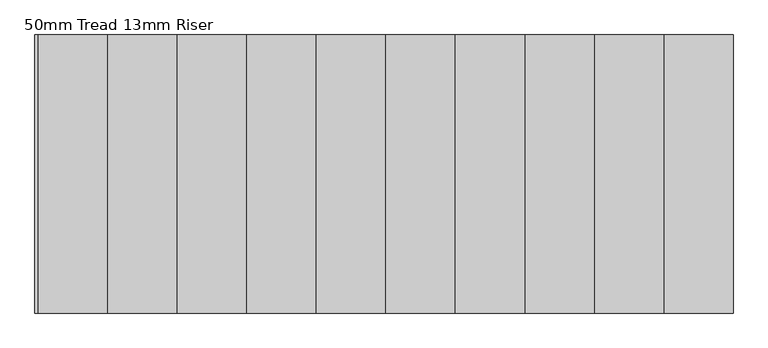
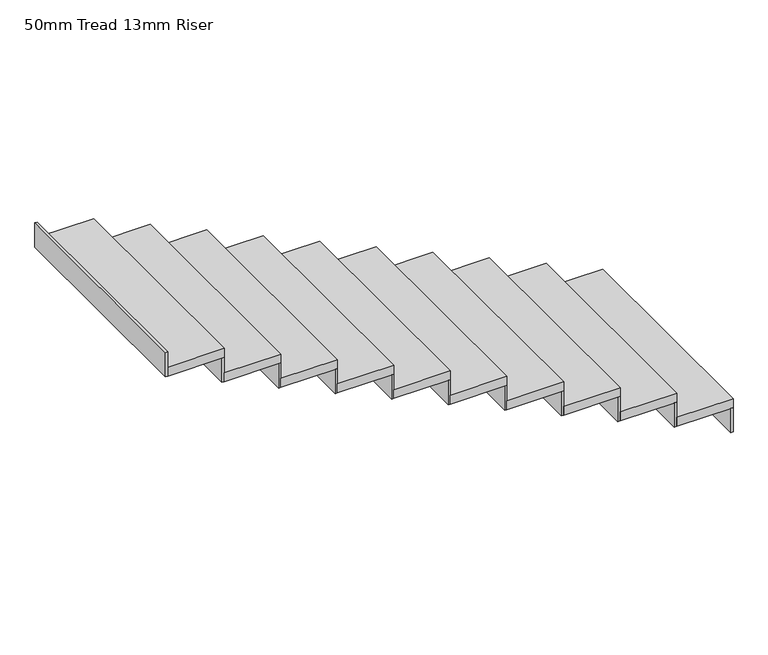
"""IFC4 building model written with IfcOpenShell, lengths in millimetres: stair flight geometry, 50mm Tread 13mm Riser."""

from ifc_helpers import new_model, si_unit, frame, origin, place, context, project, spatial, polyline, outline, extrude, source, transform, mapped, element, save


def stair_flight_50mm_tread_13mm_riser_e41575d0(model_context):
    return source(origin(), model_context, "Body", "SweptSolid", [
        extrude(outline(polyline([(20726.9907974, -2493.8863261), (20739.4907974, -2493.8863261), (20739.4907974, -3693.8863261), (20726.9907974, -3693.8863261), (20726.9907974, -2493.8863261)])), frame((0.0, 0.0, 1450.0), z_axis=(0.0, 0.0, 1.0), x_axis=(1.0, 0.0, 0.0)), (0.0, 0.0, 1.0), 136.3636364),
        extrude(outline(polyline([(20439.4907974, -3693.8863261), (20439.4907974, -2493.8863261), (20739.4907974, -2493.8863261), (20739.4907974, -3693.8863261), (20439.4907974, -3693.8863261)])), frame((0.0, 0.0, 1586.3636364), z_axis=(0.0, 0.0, 1.0), x_axis=(1.0, 0.0, 0.0)), (0.0, 0.0, 1.0), 50.0),
        extrude(outline(polyline([(20426.9907974, -2493.8863261), (20439.4907974, -2493.8863261), (20439.4907974, -3693.8863261), (20426.9907974, -3693.8863261), (20426.9907974, -2493.8863261)])), frame((0.0, 0.0, 1586.3636364), z_axis=(0.0, 0.0, 1.0), x_axis=(1.0, 0.0, 0.0)), (0.0, 0.0, 1.0), 136.3636364),
        extrude(outline(polyline([(20139.4907974, -3693.8863261), (20139.4907974, -2493.8863261), (20439.4907974, -2493.8863261), (20439.4907974, -3693.8863261), (20139.4907974, -3693.8863261)])), frame((0.0, 0.0, 1722.7272727), z_axis=(0.0, 0.0, 1.0), x_axis=(1.0, 0.0, 0.0)), (0.0, 0.0, 1.0), 50.0),
        extrude(outline(polyline([(20126.9907974, -2493.8863261), (20139.4907974, -2493.8863261), (20139.4907974, -3693.8863261), (20126.9907974, -3693.8863261), (20126.9907974, -2493.8863261)])), frame((0.0, 0.0, 1722.7272727), z_axis=(0.0, 0.0, 1.0), x_axis=(1.0, 0.0, 0.0)), (0.0, 0.0, 1.0), 136.3636364),
        extrude(outline(polyline([(19839.4907974, -3693.8863261), (19839.4907974, -2493.8863261), (20139.4907974, -2493.8863261), (20139.4907974, -3693.8863261), (19839.4907974, -3693.8863261)])), frame((0.0, 0.0, 1859.0909091), z_axis=(0.0, 0.0, 1.0), x_axis=(1.0, 0.0, 0.0)), (0.0, 0.0, 1.0), 50.0),
        extrude(outline(polyline([(19826.9907974, -2493.8863261), (19839.4907974, -2493.8863261), (19839.4907974, -3693.8863261), (19826.9907974, -3693.8863261), (19826.9907974, -2493.8863261)])), frame((0.0, 0.0, 1859.0909091), z_axis=(0.0, 0.0, 1.0), x_axis=(1.0, 0.0, 0.0)), (0.0, 0.0, 1.0), 136.3636364),
        extrude(outline(polyline([(19539.4907974, -3693.8863261), (19539.4907974, -2493.8863261), (19839.4907974, -2493.8863261), (19839.4907974, -3693.8863261), (19539.4907974, -3693.8863261)])), frame((0.0, 0.0, 1995.4545455), z_axis=(0.0, 0.0, 1.0), x_axis=(1.0, 0.0, 0.0)), (0.0, 0.0, 1.0), 50.0),
        extrude(outline(polyline([(19526.9907974, -2493.8863261), (19539.4907974, -2493.8863261), (19539.4907974, -3693.8863261), (19526.9907974, -3693.8863261), (19526.9907974, -2493.8863261)])), frame((0.0, 0.0, 1995.4545455), z_axis=(0.0, 0.0, 1.0), x_axis=(1.0, 0.0, 0.0)), (0.0, 0.0, 1.0), 136.3636364),
        extrude(outline(polyline([(19239.4907974, -3693.8863261), (19239.4907974, -2493.8863261), (19539.4907974, -2493.8863261), (19539.4907974, -3693.8863261), (19239.4907974, -3693.8863261)])), frame((0.0, 0.0, 2131.8181818), z_axis=(0.0, 0.0, 1.0), x_axis=(1.0, 0.0, 0.0)), (0.0, 0.0, 1.0), 50.0),
        extrude(outline(polyline([(19226.9907974, -2493.8863261), (19239.4907974, -2493.8863261), (19239.4907974, -3693.8863261), (19226.9907974, -3693.8863261), (19226.9907974, -2493.8863261)])), frame((0.0, 0.0, 2131.8181818), z_axis=(0.0, 0.0, 1.0), x_axis=(1.0, 0.0, 0.0)), (0.0, 0.0, 1.0), 136.3636364),
        extrude(outline(polyline([(18939.4907974, -3693.8863261), (18939.4907974, -2493.8863261), (19239.4907974, -2493.8863261), (19239.4907974, -3693.8863261), (18939.4907974, -3693.8863261)])), frame((0.0, 0.0, 2268.1818182), z_axis=(0.0, 0.0, 1.0), x_axis=(1.0, 0.0, 0.0)), (0.0, 0.0, 1.0), 50.0),
        extrude(outline(polyline([(18926.9907974, -2493.8863261), (18939.4907974, -2493.8863261), (18939.4907974, -3693.8863261), (18926.9907974, -3693.8863261), (18926.9907974, -2493.8863261)])), frame((0.0, 0.0, 2268.1818182), z_axis=(0.0, 0.0, 1.0), x_axis=(1.0, 0.0, 0.0)), (0.0, 0.0, 1.0), 136.3636364),
        extrude(outline(polyline([(18639.4907974, -3693.8863261), (18639.4907974, -2493.8863261), (18939.4907974, -2493.8863261), (18939.4907974, -3693.8863261), (18639.4907974, -3693.8863261)])), frame((0.0, 0.0, 2404.5454545), z_axis=(0.0, 0.0, 1.0), x_axis=(1.0, 0.0, 0.0)), (0.0, 0.0, 1.0), 50.0),
        extrude(outline(polyline([(18626.9907974, -2493.8863261), (18639.4907974, -2493.8863261), (18639.4907974, -3693.8863261), (18626.9907974, -3693.8863261), (18626.9907974, -2493.8863261)])), frame((0.0, 0.0, 2404.5454545), z_axis=(0.0, 0.0, 1.0), x_axis=(1.0, 0.0, 0.0)), (0.0, 0.0, 1.0), 136.3636364),
        extrude(outline(polyline([(18339.4907974, -3693.8863261), (18339.4907974, -2493.8863261), (18639.4907974, -2493.8863261), (18639.4907974, -3693.8863261), (18339.4907974, -3693.8863261)])), frame((0.0, 0.0, 2540.9090909), z_axis=(0.0, 0.0, 1.0), x_axis=(1.0, 0.0, 0.0)), (0.0, 0.0, 1.0), 50.0),
        extrude(outline(polyline([(18326.9907974, -2493.8863261), (18339.4907974, -2493.8863261), (18339.4907974, -3693.8863261), (18326.9907974, -3693.8863261), (18326.9907974, -2493.8863261)])), frame((0.0, 0.0, 2540.9090909), z_axis=(0.0, 0.0, 1.0), x_axis=(1.0, 0.0, 0.0)), (0.0, 0.0, 1.0), 136.3636364),
        extrude(outline(polyline([(18039.4907974, -3693.8863261), (18039.4907974, -2493.8863261), (18339.4907974, -2493.8863261), (18339.4907974, -3693.8863261), (18039.4907974, -3693.8863261)])), frame((0.0, 0.0, 2677.2727273), z_axis=(0.0, 0.0, 1.0), x_axis=(1.0, 0.0, 0.0)), (0.0, 0.0, 1.0), 50.0),
        extrude(outline(polyline([(18026.9907974, -2493.8863261), (18039.4907974, -2493.8863261), (18039.4907974, -3693.8863261), (18026.9907974, -3693.8863261), (18026.9907974, -2493.8863261)])), frame((0.0, 0.0, 2677.2727273), z_axis=(0.0, 0.0, 1.0), x_axis=(1.0, 0.0, 0.0)), (0.0, 0.0, 1.0), 136.3636364),
        extrude(outline(polyline([(17726.9907974, -2493.8863261), (17739.4907974, -2493.8863261), (17739.4907974, -3693.8863261), (17726.9907974, -3693.8863261), (17726.9907974, -2493.8863261)])), frame((0.0, 0.0, 2813.6363636), z_axis=(0.0, 0.0, 1.0), x_axis=(1.0, 0.0, 0.0)), (0.0, 0.0, 1.0), 136.3636364),
        extrude(outline(polyline([(17739.4907974, -3693.8863261), (17739.4907974, -2493.8863261), (18039.4907974, -2493.8863261), (18039.4907974, -3693.8863261), (17739.4907974, -3693.8863261)])), frame((0.0, 0.0, 2813.6363636), z_axis=(0.0, 0.0, 1.0), x_axis=(1.0, 0.0, 0.0)), (0.0, 0.0, 1.0), 50.0),
    ])


if __name__ == "__main__":
    model = new_model("IFC4")
    model_context = context("Model", 3, world=origin())
    ifc_project = project(units=[si_unit("LENGTHUNIT", "METRE", prefix="MILLI")], contexts=[model_context])
    site = spatial("IfcSite", under=ifc_project)
    building = spatial("IfcBuilding", under=site)
    placement = place(None, origin())
    stair_flight_50mm_tread_13mm_riser_shape = stair_flight_50mm_tread_13mm_riser_e41575d0(model_context)
    element("IfcStairFlight", 1, ObjectType="50mm Tread 13mm Riser", at=placement, inside=building, context=model_context, shape_type="MappedRepresentation", body=[
        mapped(stair_flight_50mm_tread_13mm_riser_shape, transform((0.0, 0.0, 0.0), x_axis=(1.0, 0.0, 0.0), y_axis=(0.0, 1.0, 0.0), z_axis=(0.0, 0.0, 1.0))),
    ])
    save(model, "model.ifc")
